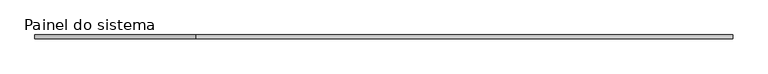
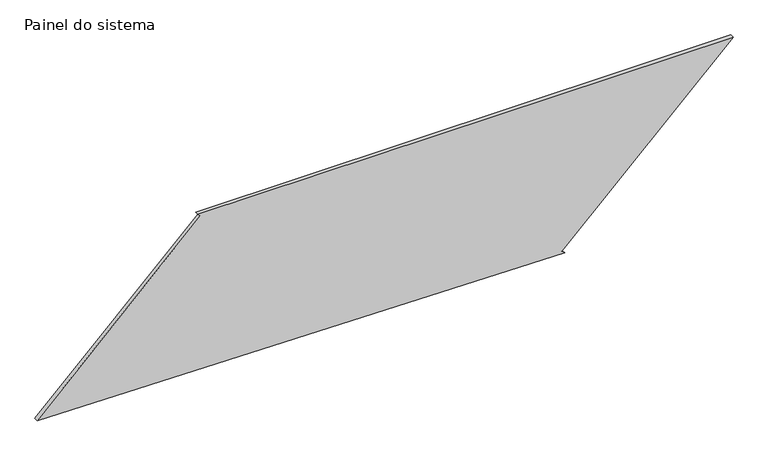
"""IFC4 building model written with IfcOpenShell, lengths in millimetres: plate geometry, Painel do sistema : Envidraçado."""

from ifc_helpers import new_model, si_unit, frame, origin, place, context, project, spatial, polyline, outline, extrude, source, transform, mapped, element, save


def painel_do_sistema_b5a43605(model_context):
    return source(origin(), model_context, "Body", "SweptSolid", [
        extrude(outline(polyline([(0.0, 1224.2150157), (17.9061609, 1206.7688298), (1154.9152222, 2373.7555523), (1154.9152222, -1276.9405954), (1137.0090613, -1259.4944096), (51.3711603, -2373.7555523), (0.0, 1224.2150157)])), frame((0.0, 24.5, 0.0), z_axis=(0.0, 1.0, 0.0), x_axis=(0.0, 0.0, 1.0)), (0.0, 0.0, 1.0), 25.0),
    ])


if __name__ == "__main__":
    model = new_model("IFC4")
    model_context = context("Model", 3, world=origin())
    ifc_project = project(units=[si_unit("LENGTHUNIT", "METRE", prefix="MILLI")], contexts=[model_context])
    site = spatial("IfcSite", under=ifc_project)
    building = spatial("IfcBuilding", under=site)
    placement = place(None, origin())
    painel_do_sistema_shape = painel_do_sistema_b5a43605(model_context)
    element("IfcPlate", 1, ObjectType="Painel do sistema : Envidraçado", at=placement, inside=building, context=model_context, shape_type="MappedRepresentation", body=[
        mapped(painel_do_sistema_shape, transform((0.0, 0.0, 0.0), x_axis=(1.0, 0.0, 0.0), y_axis=(0.0, 1.0, 0.0), z_axis=(0.0, 0.0, 1.0))),
    ])
    save(model, "model.ifc")

# Revit data of these elements
# Type "Painel do sistema : Envidraçado"
#   Construction Type Id = "GSP4R"
#   Analytic Construction = "Vidraça única Pilkington 1/8 pol"
#   Visual Light Transmittance = 0.9
#   Solar Heat Gain Coefficient = 0.86
#   Heat Transfer Coefficient (U) = 6.7069 W/(m²·K)
# Element 1 (IfcPlate, "Painel do sistema : Envidraçado")
#   Materials on its faces: "Vidro"
# Materials
#   "Vidro": class "Vidro", colour RGB 0 128 192, transparency 0.9, Description = "Vidro de sílica", Cost = 0
